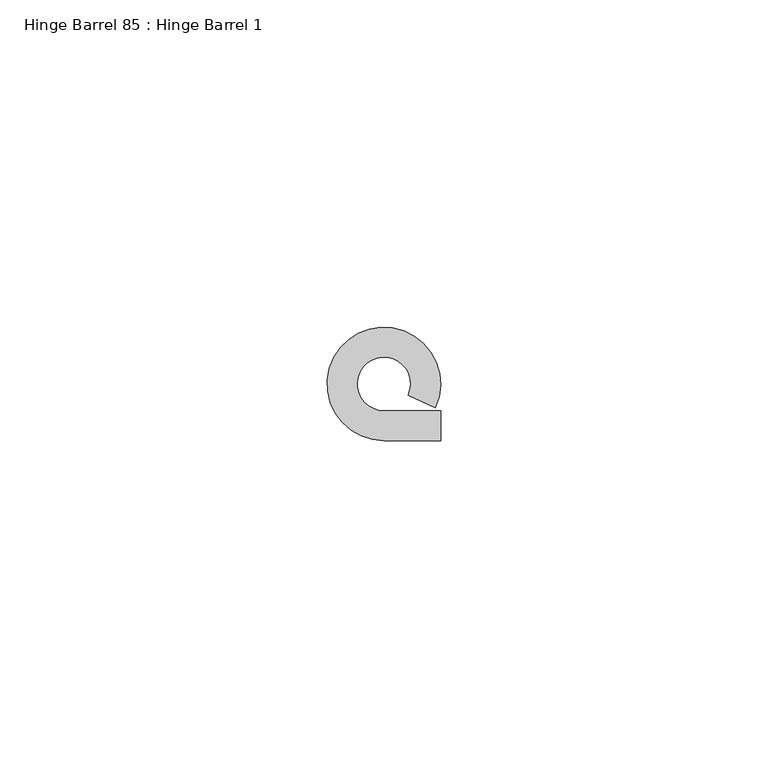
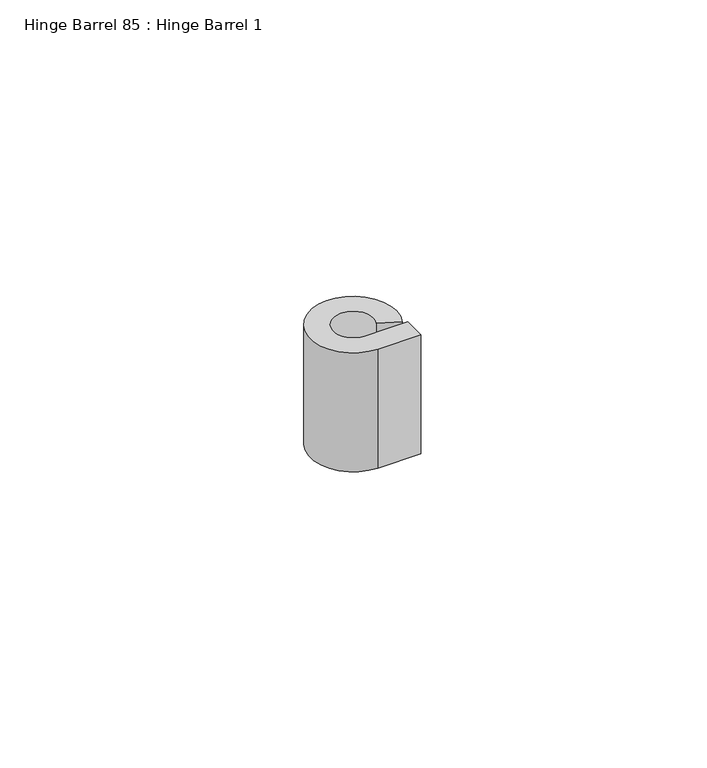
"""IFC4 building model written with IfcOpenShell, lengths in millimetres: proxy geometry, Hinge Barrel 85 : Hinge Barrel 1."""

from ifc_helpers import new_model, si_unit, point, frame, frame_2d, origin, place, context, project, spatial, polyline, circle_curve, trimmed, segment, composite_curve, outline, extrude, source, transform, mapped, element, save


def hinge_barrel_85_hinge_barrel_1_91723ac2(model_context):
    return source(origin(), model_context, "Body", "SweptSolid", [
        extrude(outline(composite_curve([segment(polyline([(587323.2214739, -531780.6943841), (587327.7934739, -531780.6943841), (587327.7934739, -531785.2584466), (587319.1320739, -531785.2584466)]), True, "CONTINUOUS"), segment(trimmed(circle_curve(frame_2d((587319.1320739, -531776.6049841)), 8.6534625), [point((587319.1320739, -531785.2584466))], [point((587326.986084, -531780.2377433))], False, "CARTESIAN"), True, "CONTINUOUS"), segment(polyline([(587326.986084, -531780.2377433), (587322.8436736, -531778.321731)]), True, "CONTINUOUS"), segment(trimmed(circle_curve(frame_2d((587319.1320739, -531776.6049841)), 4.0894), [point((587322.8436736, -531778.321731))], [point((587319.1320739, -531780.6943841))], True, "CARTESIAN"), True, "CONTINUOUS"), segment(polyline([(587319.1320739, -531780.6943841), (587323.2214739, -531780.6943841)]), True, "CONTINUOUS")], self_intersect=False)), frame((0.0, 0.0, 1123.95), z_axis=(0.0, 0.0, 1.0), x_axis=(1.0, 0.0, 0.0)), (0.0, 0.0, 1.0), 25.4),
    ])


if __name__ == "__main__":
    model = new_model("IFC4")
    model_context = context("Model", 3, world=origin())
    ifc_project = project(units=[si_unit("LENGTHUNIT", "METRE", prefix="MILLI")], contexts=[model_context])
    site = spatial("IfcSite", under=ifc_project)
    building = spatial("IfcBuilding", under=site)
    placement = place(None, origin())
    hinge_barrel_85_hinge_barrel_1_shape = hinge_barrel_85_hinge_barrel_1_91723ac2(model_context)
    element("IfcBuildingElementProxy", 1, Name="Hinge Barrel 85 : Hinge Barrel 1", ObjectType="Hinge Barrel 85 : Hinge Barrel 1", at=placement, inside=building, context=model_context, shape_type="MappedRepresentation", body=[
        mapped(hinge_barrel_85_hinge_barrel_1_shape, transform((0.0, 0.0, 0.0), x_axis=(1.0, 0.0, 0.0), y_axis=(0.0, 1.0, 0.0), z_axis=(0.0, 0.0, 1.0))),
    ])
    save(model, "model.ifc")

# Revit data of these elements
# Element 1 (IfcBuildingElementProxy, "Hinge Barrel 85 : Hinge Barrel 1")
#   Materials on its faces: "6\"X6\" WELD-ON STL BUTT HINGE"
# Materials
#   "6\"X6\" WELD-ON STL BUTT HINGE": class "Metal", colour RGB 189 187 185, transparency 0, Description = "Carbon steel", Cost = 0
